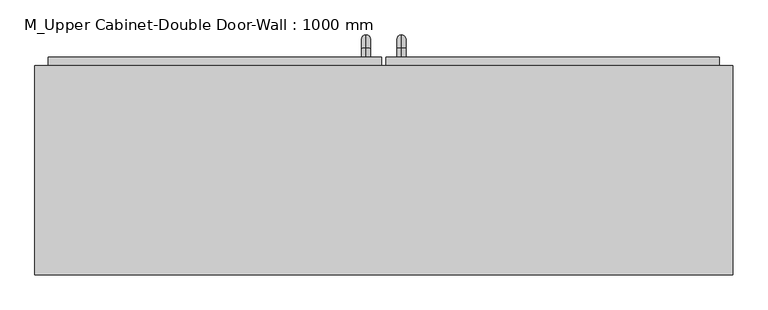
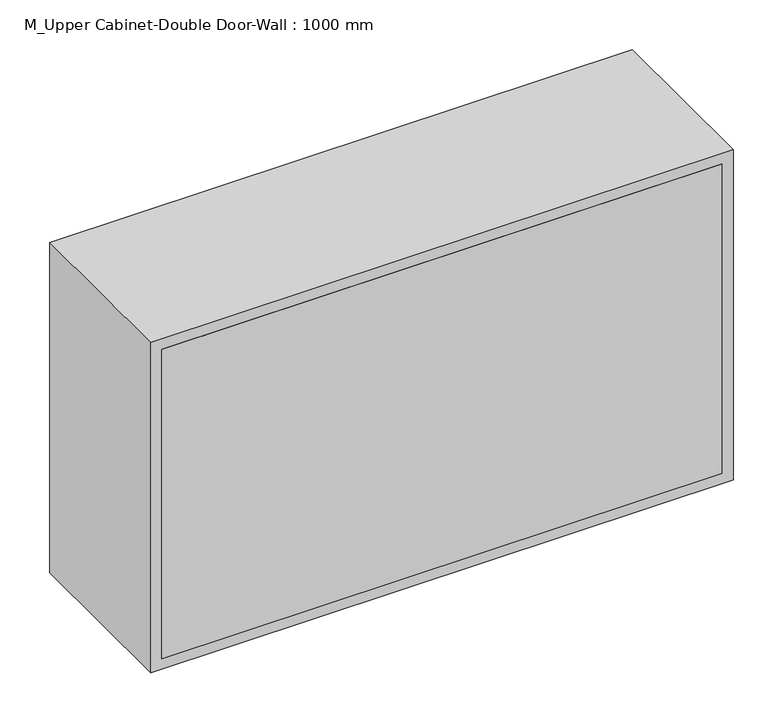
"""IFC4 building model written with IfcOpenShell, lengths in millimetres: furniture geometry, M_Upper Cabinet-Double Door-Wall : 1000 mm."""

from ifc_helpers import new_model, si_unit, point, frame, origin, place, context, project, spatial, polyline, circle_curve, ellipse_curve, trimmed, outline, extrude, source, transform, mapped, element, save
from ifc_brep_helpers import plane_surface, cylinder_surface, revolved_surface, advanced_brep


def m_upper_cabinet_double_door_wall_1000_mm_94f65b6b(model_context):
    return source(origin(), model_context, "Body", "SolidModel", [
        advanced_brep(
        [(55.1711628, 374.7, 1546.05), (55.1711628, 374.7, 1558.75), (55.1711628, 387.4, 1546.05), (55.1711628, 387.4, 1558.75), (55.1711628, 406.45, 1539.7), (55.1711628, 393.75, 1539.7), (55.1711628, 393.75, 1463.5), (55.1711628, 406.45, 1463.5), (55.1711628, 387.4, 1444.45), (55.1711628, 387.4, 1457.15), (55.1711628, 374.7, 1457.15), (55.1711628, 374.7, 1444.45)],
        [
            (0, 1, circle_curve(frame((55.1711628, 374.7, 1552.4), z_axis=(0.0, -1.0, 0.0), x_axis=(0.0, 0.0, -1.0)), 6.35)),
            (1, 0, circle_curve(frame((55.1711628, 374.7, 1552.4), z_axis=(0.0, -1.0, 0.0), x_axis=(0.0, 0.0, -1.0)), 6.35)),
            (0, 2),
            (2, 3, circle_curve(frame((55.1711628, 387.4, 1552.4), z_axis=(0.0, -1.0, 0.0), x_axis=(0.0, 0.0, -1.0)), 6.35)),
            (3, 1),
            (3, 2, circle_curve(frame((55.1711628, 387.4, 1552.4), z_axis=(0.0, -1.0, 0.0), x_axis=(0.0, 0.0, -1.0)), 6.35)),
            (4, 3, circle_curve(frame((55.1711628, 387.4, 1539.7), z_axis=(1.0, 0.0, 0.0), x_axis=(0.0, 0.0, 1.0)), 19.05)),
            (2, 5, circle_curve(frame((55.1711628, 387.4, 1539.7), z_axis=(-1.0, 0.0, 0.0), x_axis=(0.0, 0.0, 1.0)), 6.35)),
            (5, 4, circle_curve(frame((55.1711628, 400.1, 1539.7), z_axis=(0.0, 0.0, 1.0), x_axis=(0.0, -1.0, 0.0)), 6.35)),
            (4, 5, circle_curve(frame((55.1711628, 400.1, 1539.7), z_axis=(0.0, 0.0, 1.0), x_axis=(0.0, -1.0, 0.0)), 6.35)),
            (5, 6),
            (6, 7, circle_curve(frame((55.1711628, 400.1, 1463.5), z_axis=(0.0, 0.0, 1.0), x_axis=(0.0, -1.0, 0.0)), 6.35)),
            (7, 4),
            (7, 6, circle_curve(frame((55.1711628, 400.1, 1463.5), z_axis=(0.0, 0.0, 1.0), x_axis=(0.0, -1.0, 0.0)), 6.35)),
            (8, 7, circle_curve(frame((55.1711628, 387.4, 1463.5), z_axis=(1.0, 0.0, 0.0), x_axis=(0.0, 1.0, 0.0)), 19.05)),
            (6, 9, circle_curve(frame((55.1711628, 387.4, 1463.5), z_axis=(-1.0, 0.0, 0.0), x_axis=(0.0, 1.0, 0.0)), 6.35)),
            (9, 8, circle_curve(frame((55.1711628, 387.4, 1450.8), z_axis=(0.0, 1.0, 0.0), x_axis=(0.0, 0.0, 1.0)), 6.35)),
            (8, 9, circle_curve(frame((55.1711628, 387.4, 1450.8), z_axis=(0.0, 1.0, 0.0), x_axis=(0.0, 0.0, 1.0)), 6.35)),
            (10, 11, circle_curve(frame((55.1711628, 374.7, 1450.8), z_axis=(0.0, -1.0, 0.0), x_axis=(0.0, 0.0, 1.0)), 6.35)),
            (11, 10, circle_curve(frame((55.1711628, 374.7, 1450.8), z_axis=(0.0, -1.0, 0.0), x_axis=(0.0, 0.0, 1.0)), 6.35)),
            (9, 10),
            (11, 8),
        ],
        [
            plane_surface(frame((48.8211628, 374.7, 1552.4), z_axis=(0.0, -1.0, 0.0), x_axis=(0.0, 0.0, 1.0))),
            cylinder_surface(frame((55.1711628, 374.7, 1552.4), z_axis=(0.0, -1.0, 0.0), x_axis=(0.0, 0.0, -1.0)), 6.35),
            revolved_surface(trimmed(ellipse_curve(frame((55.1711628, 387.4, 1552.4), z_axis=(0.0, -1.0, 0.0), x_axis=(0.0, 0.0, -1.0)), 6.35, 6.35), [point((55.1711628, 387.4, 1546.05))], [point((55.1711628, 387.4, 1558.75))], True, "CARTESIAN"), (55.1711628, 387.4, 1539.7), (-1.0, 0.0, 0.0)),
            revolved_surface(trimmed(ellipse_curve(frame((55.1711628, 387.4, 1552.4), z_axis=(0.0, -1.0, 0.0), x_axis=(0.0, 0.0, -1.0)), 6.35, 6.35), [point((55.1711628, 387.4, 1558.75))], [point((55.1711628, 387.4, 1546.05))], True, "CARTESIAN"), (55.1711628, 387.4, 1539.7), (-1.0, 0.0, 0.0)),
            cylinder_surface(frame((55.1711628, 400.1, 1539.7), z_axis=(0.0, 0.0, 1.0), x_axis=(0.0, -1.0, 0.0)), 6.35),
            revolved_surface(trimmed(ellipse_curve(frame((55.1711628, 400.1, 1463.5), z_axis=(0.0, 0.0, 1.0), x_axis=(0.0, -1.0, 0.0)), 6.35, 6.35), [point((55.1711628, 393.75, 1463.5))], [point((55.1711628, 406.45, 1463.5))], True, "CARTESIAN"), (55.1711628, 387.4, 1463.5), (-1.0, 0.0, 0.0)),
            revolved_surface(trimmed(ellipse_curve(frame((55.1711628, 400.1, 1463.5), z_axis=(0.0, 0.0, 1.0), x_axis=(0.0, -1.0, 0.0)), 6.35, 6.35), [point((55.1711628, 406.45, 1463.5))], [point((55.1711628, 393.75, 1463.5))], True, "CARTESIAN"), (55.1711628, 387.4, 1463.5), (-1.0, 0.0, 0.0)),
            plane_surface(frame((48.8211628, 374.7, 1450.8), z_axis=(0.0, -1.0, 0.0), x_axis=(0.0, 0.0, -1.0))),
            cylinder_surface(frame((55.1711628, 387.4, 1450.8), z_axis=(0.0, 1.0, 0.0), x_axis=(0.0, 0.0, 1.0)), 6.35),
        ],
        [
            (0, [[1, 2]]),
            (1, [[-1, 3, 4, 5]]),
            (1, [[-2, -5, 6, -3]]),
            (2, [[7, -4, 8, 9]]),
            (3, [[-8, -6, -7, 10]]),
            (4, [[-9, 11, 12, 13]]),
            (4, [[-10, -13, 14, -11]]),
            (5, [[15, -12, 16, 17]]),
            (6, [[-16, -14, -15, 18]]),
            (7, [[19, 20]]),
            (8, [[-17, 21, -20, 22]]),
            (8, [[-18, -22, -19, -21]]),
        ],
    ),
        advanced_brep(
        [(4.3711628, 374.7, 1546.05), (4.3711628, 374.7, 1558.75), (4.3711628, 387.4, 1546.05), (4.3711628, 387.4, 1558.75), (4.3711628, 406.45, 1539.7), (4.3711628, 393.75, 1539.7), (4.3711628, 393.75, 1463.5), (4.3711628, 406.45, 1463.5), (4.3711628, 387.4, 1444.45), (4.3711628, 387.4, 1457.15), (4.3711628, 374.7, 1457.15), (4.3711628, 374.7, 1444.45)],
        [
            (0, 1, circle_curve(frame((4.3711628, 374.7, 1552.4), z_axis=(0.0, -1.0, 0.0), x_axis=(0.0, 0.0, 1.0)), 6.35)),
            (1, 0, circle_curve(frame((4.3711628, 374.7, 1552.4), z_axis=(0.0, -1.0, 0.0), x_axis=(0.0, 0.0, 1.0)), 6.35)),
            (0, 2),
            (2, 3, circle_curve(frame((4.3711628, 387.4, 1552.4), z_axis=(0.0, -1.0, 0.0), x_axis=(0.0, 0.0, 1.0)), 6.35)),
            (3, 1),
            (3, 2, circle_curve(frame((4.3711628, 387.4, 1552.4), z_axis=(0.0, -1.0, 0.0), x_axis=(0.0, 0.0, 1.0)), 6.35)),
            (4, 3, circle_curve(frame((4.3711628, 387.4, 1539.7), z_axis=(1.0, 0.0, 0.0), x_axis=(0.0, 0.0, 1.0)), 19.05)),
            (2, 5, circle_curve(frame((4.3711628, 387.4, 1539.7), z_axis=(-1.0, 0.0, 0.0), x_axis=(0.0, 0.0, 1.0)), 6.35)),
            (5, 4, circle_curve(frame((4.3711628, 400.1, 1539.7), z_axis=(0.0, 0.0, 1.0), x_axis=(0.0, 1.0, 0.0)), 6.35)),
            (4, 5, circle_curve(frame((4.3711628, 400.1, 1539.7), z_axis=(0.0, 0.0, 1.0), x_axis=(0.0, 1.0, 0.0)), 6.35)),
            (5, 6),
            (6, 7, circle_curve(frame((4.3711628, 400.1, 1463.5), z_axis=(0.0, 0.0, 1.0), x_axis=(0.0, 1.0, 0.0)), 6.35)),
            (7, 4),
            (7, 6, circle_curve(frame((4.3711628, 400.1, 1463.5), z_axis=(0.0, 0.0, 1.0), x_axis=(0.0, 1.0, 0.0)), 6.35)),
            (8, 7, circle_curve(frame((4.3711628, 387.4, 1463.5), z_axis=(1.0, 0.0, 0.0), x_axis=(0.0, 1.0, 0.0)), 19.05)),
            (6, 9, circle_curve(frame((4.3711628, 387.4, 1463.5), z_axis=(-1.0, 0.0, 0.0), x_axis=(0.0, 1.0, 0.0)), 6.35)),
            (9, 8, circle_curve(frame((4.3711628, 387.4, 1450.8), z_axis=(0.0, 1.0, 0.0), x_axis=(0.0, 0.0, -1.0)), 6.35)),
            (8, 9, circle_curve(frame((4.3711628, 387.4, 1450.8), z_axis=(0.0, 1.0, 0.0), x_axis=(0.0, 0.0, -1.0)), 6.35)),
            (10, 11, circle_curve(frame((4.3711628, 374.7, 1450.8), z_axis=(0.0, -1.0, 0.0), x_axis=(0.0, 0.0, -1.0)), 6.35)),
            (11, 10, circle_curve(frame((4.3711628, 374.7, 1450.8), z_axis=(0.0, -1.0, 0.0), x_axis=(0.0, 0.0, -1.0)), 6.35)),
            (9, 10),
            (11, 8),
        ],
        [
            plane_surface(frame((-1.9788372, 374.7, 1552.4), z_axis=(0.0, -1.0, 0.0), x_axis=(0.0, 0.0, 1.0))),
            cylinder_surface(frame((4.3711628, 374.7, 1552.4), z_axis=(0.0, -1.0, 0.0), x_axis=(0.0, 0.0, 1.0)), 6.35),
            revolved_surface(trimmed(ellipse_curve(frame((4.3711628, 387.4, 1552.4), z_axis=(0.0, -1.0, 0.0), x_axis=(0.0, 0.0, 1.0)), 6.35, 6.35), [point((4.3711628, 387.4, 1546.05))], [point((4.3711628, 387.4, 1558.75))], True, "CARTESIAN"), (4.3711628, 387.4, 1539.7), (-1.0, 0.0, 0.0)),
            revolved_surface(trimmed(ellipse_curve(frame((4.3711628, 387.4, 1552.4), z_axis=(0.0, -1.0, 0.0), x_axis=(0.0, 0.0, 1.0)), 6.35, 6.35), [point((4.3711628, 387.4, 1558.75))], [point((4.3711628, 387.4, 1546.05))], True, "CARTESIAN"), (4.3711628, 387.4, 1539.7), (-1.0, 0.0, 0.0)),
            cylinder_surface(frame((4.3711628, 400.1, 1539.7), z_axis=(0.0, 0.0, 1.0), x_axis=(0.0, 1.0, 0.0)), 6.35),
            revolved_surface(trimmed(ellipse_curve(frame((4.3711628, 400.1, 1463.5), z_axis=(0.0, 0.0, 1.0), x_axis=(0.0, 1.0, 0.0)), 6.35, 6.35), [point((4.3711628, 393.75, 1463.5))], [point((4.3711628, 406.45, 1463.5))], True, "CARTESIAN"), (4.3711628, 387.4, 1463.5), (-1.0, 0.0, 0.0)),
            revolved_surface(trimmed(ellipse_curve(frame((4.3711628, 400.1, 1463.5), z_axis=(0.0, 0.0, 1.0), x_axis=(0.0, 1.0, 0.0)), 6.35, 6.35), [point((4.3711628, 406.45, 1463.5))], [point((4.3711628, 393.75, 1463.5))], True, "CARTESIAN"), (4.3711628, 387.4, 1463.5), (-1.0, 0.0, 0.0)),
            plane_surface(frame((-1.9788372, 374.7, 1450.8), z_axis=(0.0, -1.0, 0.0), x_axis=(0.0, 0.0, -1.0))),
            cylinder_surface(frame((4.3711628, 387.4, 1450.8), z_axis=(0.0, 1.0, 0.0), x_axis=(0.0, 0.0, -1.0)), 6.35),
        ],
        [
            (0, [[1, 2]]),
            (1, [[-1, 3, 4, 5]]),
            (1, [[-2, -5, 6, -3]]),
            (2, [[7, -4, 8, 9]]),
            (3, [[-8, -6, -7, 10]]),
            (4, [[-9, 11, 12, 13]]),
            (4, [[-10, -13, 14, -11]]),
            (5, [[15, -12, 16, 17]]),
            (6, [[-16, -14, -15, 18]]),
            (7, [[19, 20]]),
            (8, [[-17, 21, -20, 22]]),
            (8, [[-18, -22, -19, -21]]),
        ],
    ),
        extrude(outline(polyline([(32.9461628, 374.7), (510.7211628, 374.7), (510.7211628, 342.95), (32.9461628, 342.95), (32.9461628, 374.7)])), frame((0.0, 0.0, 1419.05), z_axis=(0.0, 0.0, 1.0), x_axis=(1.0, 0.0, 0.0)), (0.0, 0.0, 1.0), 561.9),
        extrude(outline(polyline([(-451.1788372, 374.7), (26.5961628, 374.7), (26.5961628, 342.95), (-451.1788372, 342.95), (-451.1788372, 374.7)])), frame((0.0, 0.0, 1419.05), z_axis=(0.0, 0.0, 1.0), x_axis=(1.0, 0.0, 0.0)), (0.0, 0.0, 1.0), 561.9),
        extrude(outline(polyline([(510.7211628, 62.0), (-451.1788372, 62.0), (-451.1788372, 81.05), (510.7211628, 81.05), (510.7211628, 62.0)])), frame((0.0, 0.0, 1419.05), z_axis=(0.0, 0.0, 1.0), x_axis=(1.0, 0.0, 0.0)), (0.0, 0.0, 1.0), 561.9),
        extrude(outline(polyline([(2000.0, -470.2288372), (1400.0, -470.2288372), (1400.0, 529.7711628), (2000.0, 529.7711628), (2000.0, -470.2288372)]), holes=[polyline([(1980.95, -451.1788372), (1980.95, 510.7211628), (1419.05, 510.7211628), (1419.05, -451.1788372), (1980.95, -451.1788372)])]), frame((0.0, 62.0, 0.0), z_axis=(0.0, 1.0, 0.0), x_axis=(0.0, 0.0, 1.0)), (0.0, 0.0, 1.0), 300.0),
    ])


if __name__ == "__main__":
    model = new_model("IFC4")
    model_context = context("Model", 3, world=origin())
    ifc_project = project(units=[si_unit("LENGTHUNIT", "METRE", prefix="MILLI")], contexts=[model_context])
    site = spatial("IfcSite", under=ifc_project)
    building = spatial("IfcBuilding", under=site)
    placement = place(None, origin())
    m_upper_cabinet_double_door_wall_1000_mm_shape = m_upper_cabinet_double_door_wall_1000_mm_94f65b6b(model_context)
    element("IfcFurniture", 1, ObjectType="M_Upper Cabinet-Double Door-Wall : 1000 mm", at=placement, inside=building, context=model_context, shape_type="MappedRepresentation", body=[
        mapped(m_upper_cabinet_double_door_wall_1000_mm_shape, transform((0.0, 0.0, 0.0), x_axis=(1.0, 0.0, 0.0), y_axis=(0.0, 1.0, 0.0), z_axis=(0.0, 0.0, 1.0))),
    ])
    save(model, "model.ifc")

# Revit data of these elements
# Type "M_Upper Cabinet-Double Door-Wall : 1000 mm"
#   Manufacturer = "Manufacturer"
#   Finish = "Finish"
#   Construction Type = "Construction Type"
#   AccessibilityPerformance = "AccessibilityPerformance"
#   CodePerformance = "CodePerformance"
#   Area = "Area"
#   Color = "Color"
#   Constituents = "Constituents"
#   Features = "Features"
#   Finish = "Finish"
#   Grade = "Grade"
#   Material = "Material"
#   ModelReference = "ModelReference"
#   NominalHeight = "NominalHeight"
#   NominalLength = "NominalLength"
#   NominalWidth = "NominalWidth"
#   ProductionYear = "ProductionYear"
#   Reference = "Reference"
#   Shape = "Shape"
#   Size = "Size"
#   SustainabilityPerformance = "SustainabilityPerformance"
#   WarrantyDescription = "WarrantyDescription"
#   WarrantyDurationLabor = "WarrantyDurationLabor"
#   WarrantyDurationParts = "WarrantyDurationParts"
#   WarrantyGuarantorLabor = "WarrantyGuarantorLabor"
#   WarrantyGuarantorParts = "WarrantyGuarantorParts"
#   ExpectedLife = "ExpectedLife"
#   ReplacementCost = "ReplacementCost"
#   AssetAccountingType = "FIXED"
#   ModelLabel = "ModelLabel"
#   Depth = 0.300 m
#   Height = 0.600 m
#   Top Of Cabinet = 2.000 m
#   Width = 1.000 m
#   Cabinet Material = none
#   Door/Drawer Material = none
#   Handle Material = Cabinets - Handles
# Element 1 (IfcFurniture, "M_Upper Cabinet-Double Door-Wall : 1000 mm")
#   Materials on its faces: "Cabinets", "Cabinets - Handles"
# Materials
#   "Cabinets - Handles": class "Metal", colour RGB 57 57 57, transparency 0
#   "Cabinets": class "Miscellaneous", colour RGB 249 249 249, transparency 0
